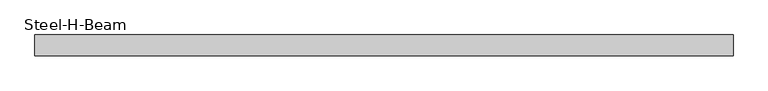
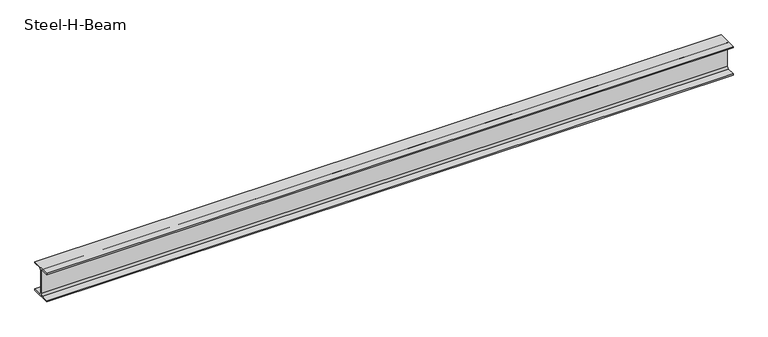
"""IFC4 building model written with IfcOpenShell, lengths in millimetres: beam geometry, Steel-H-Beam : BM121_H-294×200x8x12."""

from ifc_helpers import new_model, si_unit, point, frame, frame_2d, origin, place, context, project, spatial, polyline, circle_curve, trimmed, segment, composite_curve, outline, extrude, source, transform, mapped, element, save


def steel_h_beam_f4173fa8(model_context):
    return source(origin(), model_context, "Body", "SweptSolid", [
        extrude(outline(composite_curve([segment(polyline([(100.0, -135.0), (100.0, -147.0), (-100.0, -147.0), (-100.0, -135.0), (-22.0, -135.0)]), True, "CONTINUOUS"), segment(trimmed(circle_curve(frame_2d((-22.0, -117.0)), 18.0), [point((-22.0, -135.0))], [point((-4.0, -117.0))], True, "CARTESIAN"), True, "CONTINUOUS"), segment(polyline([(-4.0, -117.0), (-4.0, 117.0)]), True, "CONTINUOUS"), segment(trimmed(circle_curve(frame_2d((-22.0, 117.0)), 18.0), [point((-4.0, 117.0))], [point((-22.0, 135.0))], True, "CARTESIAN"), True, "CONTINUOUS"), segment(polyline([(-22.0, 135.0), (-100.0, 135.0), (-100.0, 147.0), (100.0, 147.0), (100.0, 135.0), (22.0, 135.0)]), True, "CONTINUOUS"), segment(trimmed(circle_curve(frame_2d((22.0, 117.0)), 18.0), [point((22.0, 135.0))], [point((4.0, 117.0))], True, "CARTESIAN"), True, "CONTINUOUS"), segment(polyline([(4.0, 117.0), (4.0, -117.0)]), True, "CONTINUOUS"), segment(trimmed(circle_curve(frame_2d((22.0, -117.0)), 18.0), [point((4.0, -117.0))], [point((22.0, -135.0))], True, "CARTESIAN"), True, "CONTINUOUS"), segment(polyline([(22.0, -135.0), (100.0, -135.0)]), True, "CONTINUOUS")], self_intersect=False)), frame((-3361.3486745, 0.0, 0.0), z_axis=(1.0, 0.0, 0.0), x_axis=(0.0, 1.0, 0.0)), (0.0, 0.0, 1.0), 6724.6),
    ])


if __name__ == "__main__":
    model = new_model("IFC4")
    model_context = context("Model", 3, world=origin())
    ifc_project = project(units=[si_unit("LENGTHUNIT", "METRE", prefix="MILLI")], contexts=[model_context])
    site = spatial("IfcSite", under=ifc_project)
    building = spatial("IfcBuilding", under=site)
    placement = place(None, origin())
    steel_h_beam_shape = steel_h_beam_f4173fa8(model_context)
    element("IfcBeam", 1, ObjectType="Steel-H-Beam : BM121_H-294×200x8x12", at=placement, inside=building, context=model_context, shape_type="MappedRepresentation", body=[
        mapped(steel_h_beam_shape, transform((0.0, 0.0, 0.0), x_axis=(1.0, 0.0, 0.0), y_axis=(0.0, 1.0, 0.0), z_axis=(0.0, 0.0, 1.0))),
    ])
    save(model, "model.ifc")

# Revit data of these elements
# Type "Steel-H-Beam : BM121_H-294×200x8x12"
#   Surface Area = 1.3411 m²/m
#   Section Area = 72.3812 cm²
#   Mass per Unit Length = 56.8193 kg/m
#   Length [instance default] = 3000 mm
#   B = 200 mm
#   H = 294 mm
#   r = 18 mm
#   tw = 8 mm
#   tf = 12 mm
#   hec_material4 [instance default] = none
#   hec_material3 [instance default] = none
#   hec_material2 [instance default] = none
#   hec_material1 [instance default] = none
#   Structural Material [instance default] = Steel, 45-345
#   Assembly Code = ""
# Element 1 (IfcBeam, "Steel-H-Beam : BM121_H-294×200x8x12")
#   hec_material3 = F01AC000-00002_Building/Shelter Fire Proofing Work_Intumescent Coating Type_1 hr. rating (UL 1709))
#   hec_material2 = S01AA010-00002_Main Steel Structure Fabrication Work_Shelter/Building_Steel Painting/Coating_for Fireproofed Steel Surface, Surface Preparation & Primer Coat
#   hec_material1 = S03AA028-00001_Main Steel Structure Erection Work_Shelter/Building_Medium Steel
#   Structural Material = S01AA002-00001_Main Steel Structure Fabrication Work_Shelter/Building_Medium Steel - Standard
#   Materials on its faces: "S01AA002-00001_Main Steel Structure Fabrication Work_Shelter/Building_Medium Steel - Standard"
# Materials
#   "Steel, 45-345": class "Metal", colour RGB 189 187 185, transparency 0, Description = "Steel 345 MPa", Cost = 0
#   "S01AA002-00001_Main Steel Structure Fabrication Work_Shelter/Building_Medium Steel - Standard": class "Metal", colour RGB 120 120 120, transparency 0, Comments = "(90KG/M>Weight≥30KG/M)", Description = "Structural steel 50ksi", W00) Work Master Code = "S01AA002-0001", W01) Work Master_Lv1 = "Main Steel Structure Fabrication Work", W02) Work Master_Lv2 = "Shelter/Building", W03) Work Master_Spec.1 = "Medium Steel - Standard (90KG/M>Weight≥30KG/M)", Cost = 0
#   "F01AC000-00002_Building/Shelter Fire Proofing Work_Intumescent Coating Type_1 hr. rating (UL 1709))": class "Metal", colour RGB 255 128 128, transparency 0, Description = "Paint finished steel", W00) Work Master Code = "F01AC000-00002", W01) Work Master_Lv1 = "Building/Shelter Fire Proofing Work", W02) Work Master_Lv2 = "Intumescent Coating Type", W03) Work Master_Spec.1 = "1 hr. rating (UL 1709)", Cost = 0
#   "S01AA010-00002_Main Steel Structure Fabrication Work_Shelter/Building_Steel Painting/Coating_for Fireproofed Steel Surface, Surface Preparation & Primer Coat": class "Metal", colour RGB 120 120 120, transparency 0, Description = "Paint finished steel", W00) Work Master Code = "SS01AA010-00002", W01) Work Master_Lv1 = "Main Steel Structure Fabrication Work", W02) Work Master_Lv2 = "Shelter/Building", W03) Work Master_Spec.1 = "Steel Painting/Coating", W04) Work Master_Spec.2 = "for Fireproofed Steel Surface, Surface Preparation & Primer Coat", Cost = 0
#   "S03AA028-00001_Main Steel Structure Erection Work_Shelter/Building_Medium Steel": class "Metal", colour RGB 120 120 120, transparency 0, Comments = "(90KG/M>Weight≥30KG/M)", Description = "Structural steel 50ksi", W00) Work Master Code = "S03AA028-0001", W01) Work Master_Lv1 = "Main Steel Structure Erection Work", W02) Work Master_Lv2 = "Shelter/Building", W03) Work Master_Spec.1 = "Medium Steel (90KG/M>Weight≥30KG/M)", Cost = 0
